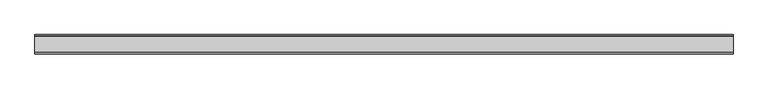
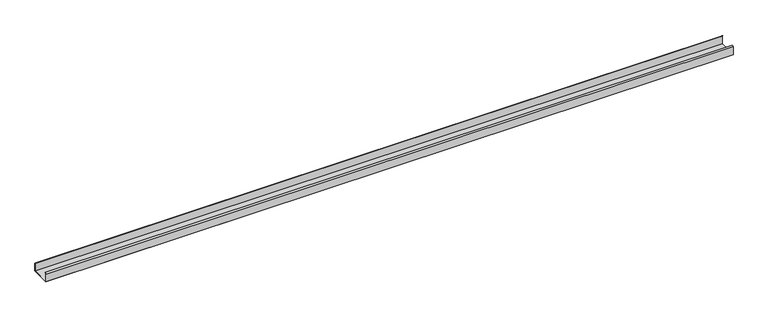
"""IFC4 building model written with IfcOpenShell, lengths in millimetres: proxy geometry, Generic Models 7:Generic Models 1:1:Generic Models 1:1 : Generic Models 7:Generic Models 1:337419:2 : Generic Models 7:Generic Models 1:1:Generic Models 1:1 : Generic Models 7:Generic Models 1:337419:306201."""

import ifcopenshell
import ifcopenshell.guid

model = None  # the IFC model being written
_history = None  # IfcOwnerHistory: only IFC2X3 demands one
_inside = {}  # id of a spatial element -> (the spatial element, [elements in it])
_under = {}  # id of a project, library or spatial element -> (it, [spatial elements below it])
_declared = {}  # id of a project -> (the project, [libraries it declares])
_typed = {}  # id of a type object -> (the type object, [elements of that type])
_made_of = {}  # id of a material, layer set ... -> (it, [elements and type objects made of it])


def new_model(schema):
    """Start an empty IFC model of exactly this schema.

    Asked for "IFC4X3", IfcOpenShell would pick the latest addendum, in which some entities
    have other attributes; the version numbers below select the first issue.
    IFC2X3 requires an IfcOwnerHistory on every rooted entity: one is made here for all.
    """
    global model, _history
    if schema == "IFC4X3":
        model = ifcopenshell.file(schema_version=(4, 3, 0, 0))
    else:
        model = ifcopenshell.file(schema=schema)
    _inside.clear()
    _under.clear()
    _declared.clear()
    _typed.clear()
    _made_of.clear()
    _history = None
    if model.schema == "IFC2X3":
        org = make("IfcOrganization", Name="unknown")
        user = make(
            "IfcPersonAndOrganization",
            ThePerson=make("IfcPerson", FamilyName="unknown"),
            TheOrganization=org,
        )
        app = make(
            "IfcApplication",
            ApplicationDeveloper=org,
            Version="unknown",
            ApplicationFullName="unknown",
            ApplicationIdentifier="unknown",
        )
        _history = make(
            "IfcOwnerHistory",
            OwningUser=user,
            OwningApplication=app,
            ChangeAction="ADDED",
            CreationDate=0,
        )
    return model


def make(cls, **values):
    """One entity of the class cls with the attributes given. An attribute that is None is left unset."""
    return model.create_entity(
        cls, **{name: value for name, value in values.items() if value is not None}
    )


def rooted(cls, **values):
    """An entity with a GlobalId (a new one), such as an element, a storey or a relation."""
    return make(cls, GlobalId=ifcopenshell.guid.new(), OwnerHistory=_history, **values)


def si_unit(unit_type, name, prefix=None):
    """IfcSIUnit, for example si_unit("LENGTHUNIT", "METRE", prefix="MILLI")."""
    return make("IfcSIUnit", UnitType=unit_type, Prefix=prefix, Name=name)


def assignment(units):
    """IfcUnitAssignment: the units of a project."""
    return None if units is None else make("IfcUnitAssignment", Units=units)


def point(xyz):
    """IfcCartesianPoint."""
    return None if xyz is None else make("IfcCartesianPoint", Coordinates=xyz)


def direction(xyz):
    """IfcDirection."""
    return None if xyz is None else make("IfcDirection", DirectionRatios=xyz)


def frame(location, z_axis=None, x_axis=None):
    """IfcAxis2Placement3D, a coordinate frame: its origin and axes. An axis left out is left unset."""
    return make(
        "IfcAxis2Placement3D",
        Location=point(location),
        Axis=direction(z_axis),
        RefDirection=direction(x_axis),
    )


def origin():
    """The frame at (0, 0, 0) with its axes left unset."""
    return frame((0.0, 0.0, 0.0))


def place(relative_to, where):
    """IfcLocalPlacement: puts the frame where relative to a parent placement (None: the world)."""
    return make(
        "IfcLocalPlacement", PlacementRelTo=relative_to, RelativePlacement=where
    )


def context(
    kind, dimensions, precision=None, world=None, true_north=None, identifier=None
):
    """IfcGeometricRepresentationContext, for example the 3D "Model" context."""
    return make(
        "IfcGeometricRepresentationContext",
        ContextIdentifier=identifier,
        ContextType=kind,
        CoordinateSpaceDimension=dimensions,
        Precision=precision,
        WorldCoordinateSystem=world,
        TrueNorth=true_north,
    )


def project(units=None, contexts=None):
    """IfcProject with its units and contexts."""
    return rooted(
        "IfcProject",
        Name="project",
        RepresentationContexts=contexts,
        UnitsInContext=assignment(units),
    )


def spatial(cls, under=None, at=None, **own):
    """A site, building, storey or space (cls), placed at a placement, below another one or the project."""
    s = rooted(cls, ObjectPlacement=at, **own)
    if under is not None:
        _under.setdefault(under.id(), (under, []))[1].append(s)
    return s


def polyline(points):
    """IfcPolyline through the points."""
    return make("IfcPolyline", Points=[point(p) for p in points])


def outline(outer, holes=None, kind="AREA"):
    """IfcArbitraryClosedProfileDef: a profile drawn as a closed curve; with holes, ...WithVoids."""
    if holes is None:
        return make("IfcArbitraryClosedProfileDef", ProfileType=kind, OuterCurve=outer)
    return make(
        "IfcArbitraryProfileDefWithVoids",
        ProfileType=kind,
        OuterCurve=outer,
        InnerCurves=holes,
    )


def extrude(swept, where, along, depth):
    """IfcExtrudedAreaSolid: the profile swept, set in the frame where, extruded along a direction by depth."""
    return make(
        "IfcExtrudedAreaSolid",
        SweptArea=swept,
        Position=where,
        ExtrudedDirection=direction(along),
        Depth=depth,
    )


def shape(context_of_items, identifier, shape_type, items):
    """IfcShapeRepresentation: the items that make up one representation, for example the "Body"."""
    return make(
        "IfcShapeRepresentation",
        ContextOfItems=context_of_items,
        RepresentationIdentifier=identifier,
        RepresentationType=shape_type,
        Items=items,
    )


def source(mapping_origin, context_of_items, identifier, shape_type, items):
    """IfcRepresentationMap: a shape defined once, which mapped items show again and again."""
    return make(
        "IfcRepresentationMap",
        MappingOrigin=mapping_origin,
        MappedRepresentation=shape(context_of_items, identifier, shape_type, items),
    )


def transform(
    local_origin,
    x_axis=None,
    y_axis=None,
    z_axis=None,
    scale=None,
    scale2=None,
    scale3=None,
    uniform=True,
):
    """IfcCartesianTransformationOperator3D, or its non-uniform kind. x_axis, y_axis, z_axis: its Axis1, 2, 3."""
    if uniform:
        return make(
            "IfcCartesianTransformationOperator3D",
            Axis1=direction(x_axis),
            Axis2=direction(y_axis),
            LocalOrigin=point(local_origin),
            Scale=scale,
            Axis3=direction(z_axis),
        )
    return make(
        "IfcCartesianTransformationOperator3DnonUniform",
        Axis1=direction(x_axis),
        Axis2=direction(y_axis),
        LocalOrigin=point(local_origin),
        Scale=scale,
        Axis3=direction(z_axis),
        Scale2=scale2,
        Scale3=scale3,
    )


def mapped(mapping_source, mapping_target):
    """IfcMappedItem: shows the shape of a source again, moved by a transform."""
    return make(
        "IfcMappedItem", MappingSource=mapping_source, MappingTarget=mapping_target
    )


def made_of(thing, what):
    """Note that an element or type object is made of a material, layer set ...; save() writes the relation."""
    if what is not None:
        _made_of.setdefault(what.id(), (what, []))[1].append(thing)
    return thing


def element(
    cls,
    number,
    at=None,
    inside=None,
    cuts=None,
    type_object=None,
    material=None,
    context=None,
    identifier="Body",
    shape_type=None,
    held_by="IfcProductDefinitionShape",
    body=None,
    shapes=None,
    **own,
):
    """One element of the class cls, such as IfcWall. Its Tag is "e" and its number.

    at: its placement. inside: the storey or other place that contains it. cuts: it is an
    opening in that element (IfcRelVoidsElement). A single representation is given by context,
    identifier, shape_type and body (its items); several are given by shapes. held_by: the class
    of the entity that holds the representations. save() writes the other relations.
    """
    e = rooted(cls, Tag="e%d" % number, ObjectPlacement=at, **own)
    if body is not None:
        shapes = [shape(context, identifier, shape_type, body)]
    if shapes is not None:
        e.Representation = make(held_by, Representations=shapes)
    if inside is not None:
        _inside.setdefault(inside.id(), (inside, []))[1].append(e)
    if cuts is not None:
        rooted(
            "IfcRelVoidsElement", RelatingBuildingElement=cuts, RelatedOpeningElement=e
        )
    if type_object is not None:
        _typed.setdefault(type_object.id(), (type_object, []))[1].append(e)
    return made_of(e, material)


def aggregate(whole, parts):
    """IfcRelAggregates: a whole, such as a stair, and the parts it consists of."""
    return rooted("IfcRelAggregates", RelatingObject=whole, RelatedObjects=parts)


def save(model, path):
    """Write the relations noted so far, then the file.

    IfcRelAggregates (storeys below a building ...), IfcRelContainedInSpatialStructure (elements
    in a storey), IfcRelDefinesByType, IfcRelAssociatesMaterial and IfcRelDeclares: one each for
    every whole, place, type object, material and project.
    """
    for whole, parts in _under.values():
        aggregate(whole, parts)
    for where, things in _inside.values():
        rooted(
            "IfcRelContainedInSpatialStructure",
            RelatedElements=things,
            RelatingStructure=where,
        )
    for kind, things in _typed.values():
        rooted("IfcRelDefinesByType", RelatedObjects=things, RelatingType=kind)
    for what, things in _made_of.values():
        rooted("IfcRelAssociatesMaterial", RelatedObjects=things, RelatingMaterial=what)
    for by, libraries in _declared.values():
        rooted("IfcRelDeclares", RelatingContext=by, RelatedDefinitions=libraries)
    model.write(path)


def generic_models_f69d2429(model_context):
    return source(origin(), model_context, "Body", "SweptSolid", [
        extrude(outline(polyline([(-578797.4913841, 3675.0625), (-579000.6913841, 3675.0625), (-579000.6913841, 3763.9625), (-578986.0982375, 3776.207604), (-578984.3124931, 3774.0794367), (-578997.9132591, 3762.667039), (-578997.9132591, 3677.840625), (-578800.2695091, 3677.840625), (-578800.2695091, 3762.667039), (-578813.8702751, 3774.0794367), (-578812.0845307, 3776.207604), (-578797.4913841, 3763.9625), (-578797.4913841, 3675.0625)])), frame((565582.1867239, 0.0, 0.0), z_axis=(1.0, 0.0, 0.0), x_axis=(0.0, 1.0, 0.0)), (0.0, 0.0, 1.0), 7315.2),
    ])


if __name__ == "__main__":
    model = new_model("IFC4")
    model_context = context("Model", 3, world=origin())
    ifc_project = project(units=[si_unit("LENGTHUNIT", "METRE", prefix="MILLI")], contexts=[model_context])
    site = spatial("IfcSite", under=ifc_project)
    building = spatial("IfcBuilding", under=site)
    placement = place(None, origin())
    generic_models_shape = generic_models_f69d2429(model_context)
    element("IfcBuildingElementProxy", 1, Name="Generic Models 7:Generic Models 1:1:Generic Models 1:1 : Generic Models 7:Generic Models 1:337419:2 : Generic Models 7:Generic Models 1:1:Generic Models 1:1 : Generic Models 7:Generic Models 1:337419:306201", ObjectType="Generic Models 7:Generic Models 1:1:Generic Models 1:1 : Generic Models 7:Generic Models 1:337419:2 : Generic Models 7:Generic Models 1:1:Generic Models 1:1 : Generic Models 7:Generic Models 1:337419:306201", at=placement, inside=building, context=model_context, shape_type="MappedRepresentation", body=[
        mapped(generic_models_shape, transform((0.0, 0.0, 0.0), x_axis=(1.0, 0.0, 0.0), y_axis=(0.0, 1.0, 0.0), z_axis=(0.0, 0.0, 1.0))),
    ])
    save(model, "model.ifc")

# Revit data of these elements
# Type "Generic Models 7:Generic Models 1:1:Generic Models 1:1 : Generic Models 7:Generic Models 1:337419:2 : Generic Models 7:Generic Models 1:1:Generic Models 1:1 : Generic Models 7:Generic Models 1:337419:306201"
#   NameOverride = "Generic Models 7:Generic Models 1:1:Generic Models 1:1 : Generic Models 7:Generic Models 1:337419:306201"
#   ObjectTypeOverride = "Generic Models 1:1 : Generic Models 7:Generic Models 1:337419"
#   Reference = "Generic Models 1"
#   Tag = "306201"
# Element 1 (IfcBuildingElementProxy, "Generic Models 7:Generic Models 1:1:Generic Models 1:1 : Generic Models 7:Generic Models 1:337419:2 : Generic Models 7:Generic Models 1:1:Generic Models 1:1 : Generic Models 7:Generic Models 1:337419:306201")
#   Materials on its faces: "'ZEE' SECTION (8.0x3.5Z - SEE STRUCT. DWGS)"
# Materials
#   "'ZEE' SECTION (8.0x3.5Z - SEE STRUCT. DWGS)": class "Unassigned", colour RGB 210 209 208, transparency 0, Keynote = "M05121300.02", Cost = 0
